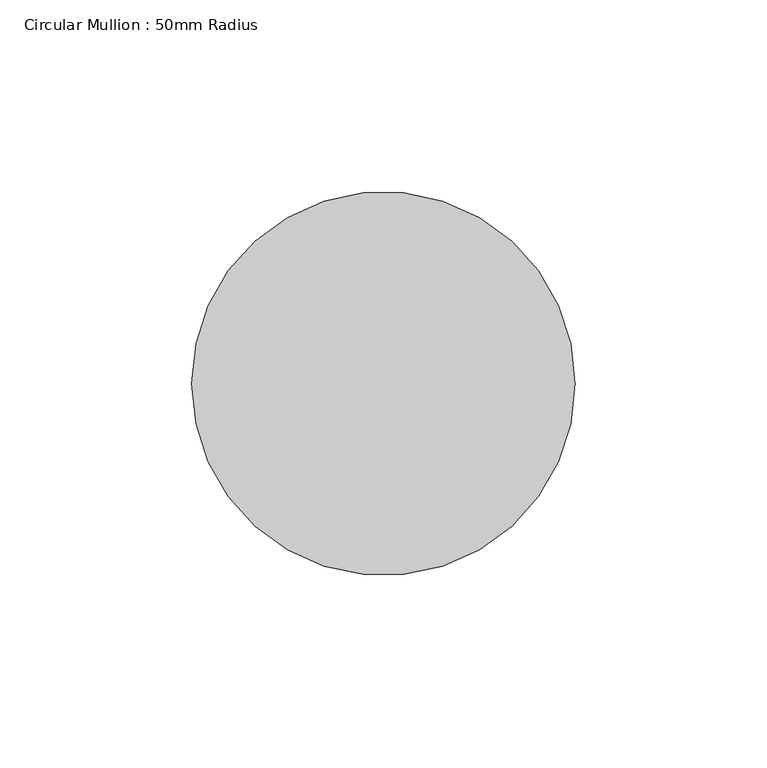
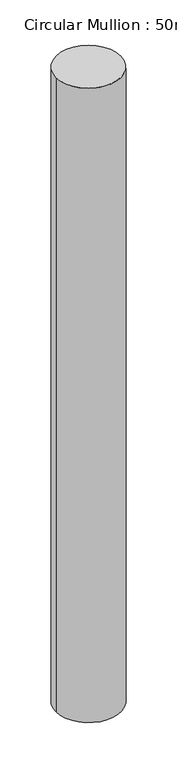
"""IFC4 building model written with IfcOpenShell, lengths in millimetres: member geometry, Circular Mullion : 50mm Radius."""

from ifc_helpers import new_model, si_unit, point, frame, origin, origin_2d, place, context, project, spatial, circle_curve, trimmed, segment, composite_curve, outline, extrude, source, transform, mapped, element, save


def circular_mullion_50mm_radius_18f620de(model_context):
    return source(origin(), model_context, "Body", "SweptSolid", [
        extrude(outline(composite_curve([segment(trimmed(circle_curve(origin_2d(), 50.0), [point((50.0, 0.0))], [point((-50.0, 0.0))], False, "CARTESIAN"), True, "CONTINUOUS"), segment(trimmed(circle_curve(origin_2d(), 50.0), [point((-50.0, 0.0))], [point((50.0, 0.0))], False, "CARTESIAN"), True, "CONTINUOUS")], self_intersect=False)), frame((0.0, 0.0, -1033.7080304), z_axis=(0.0, 0.0, 1.0), x_axis=(1.0, 0.0, 0.0)), (0.0, 0.0, 1.0), 1033.7080304),
    ])


if __name__ == "__main__":
    model = new_model("IFC4")
    model_context = context("Model", 3, world=origin())
    ifc_project = project(units=[si_unit("LENGTHUNIT", "METRE", prefix="MILLI")], contexts=[model_context])
    site = spatial("IfcSite", under=ifc_project)
    building = spatial("IfcBuilding", under=site)
    placement = place(None, origin())
    circular_mullion_50mm_radius_shape = circular_mullion_50mm_radius_18f620de(model_context)
    element("IfcMember", 1, ObjectType="Circular Mullion : 50mm Radius", at=placement, inside=building, context=model_context, shape_type="MappedRepresentation", body=[
        mapped(circular_mullion_50mm_radius_shape, transform((0.0, 0.0, 0.0), x_axis=(1.0, 0.0, 0.0), y_axis=(0.0, 1.0, 0.0), z_axis=(0.0, 0.0, 1.0))),
    ])
    save(model, "model.ifc")

# Revit data of these elements
# Type "Circular Mullion : 50mm Radius"
#   built-in parameter 1007350 = 0.164042 (stored number, unit not read)
# Element 1 (IfcMember, "Circular Mullion : 50mm Radius")
#   Materials on its faces: "Aluminium"
# Materials
#   "Aluminium": class "Metal", colour RGB 247 247 247, transparency 0, Description = "Aluminium 6061", Cost = 0
